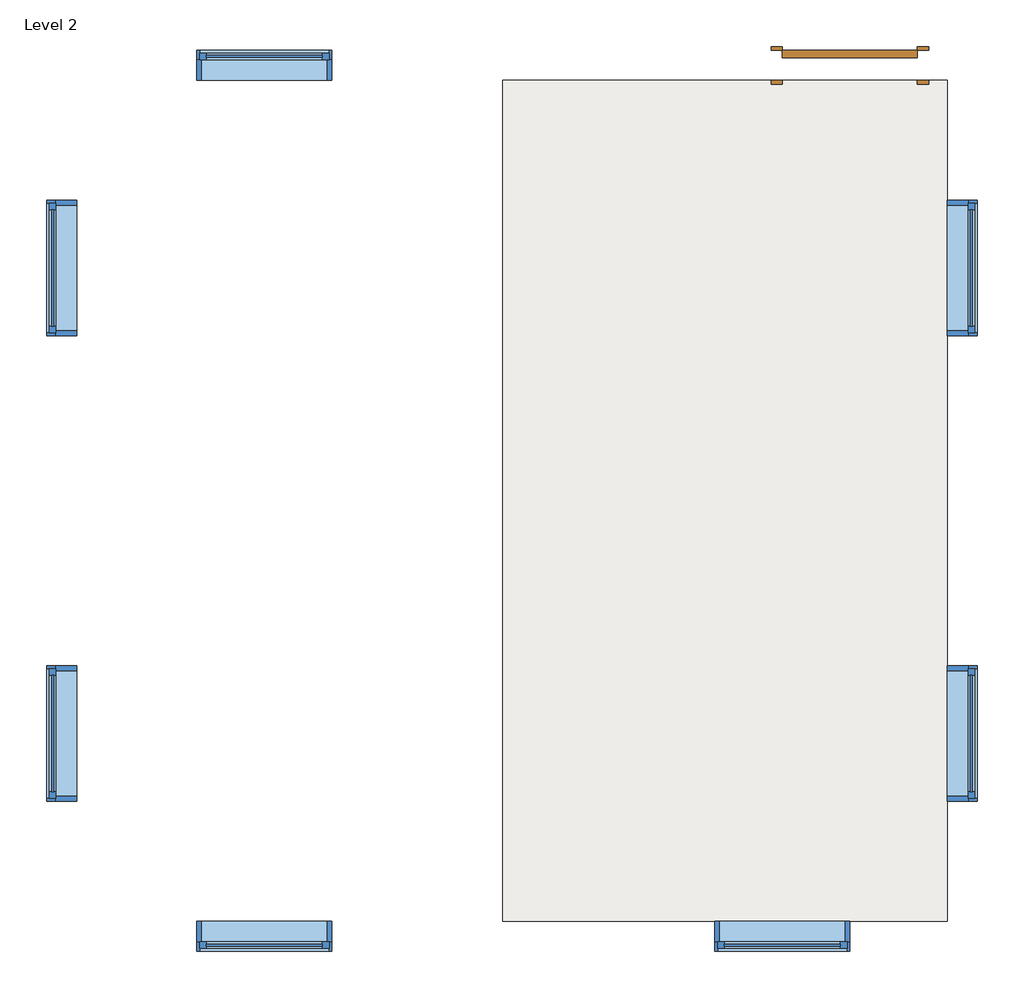
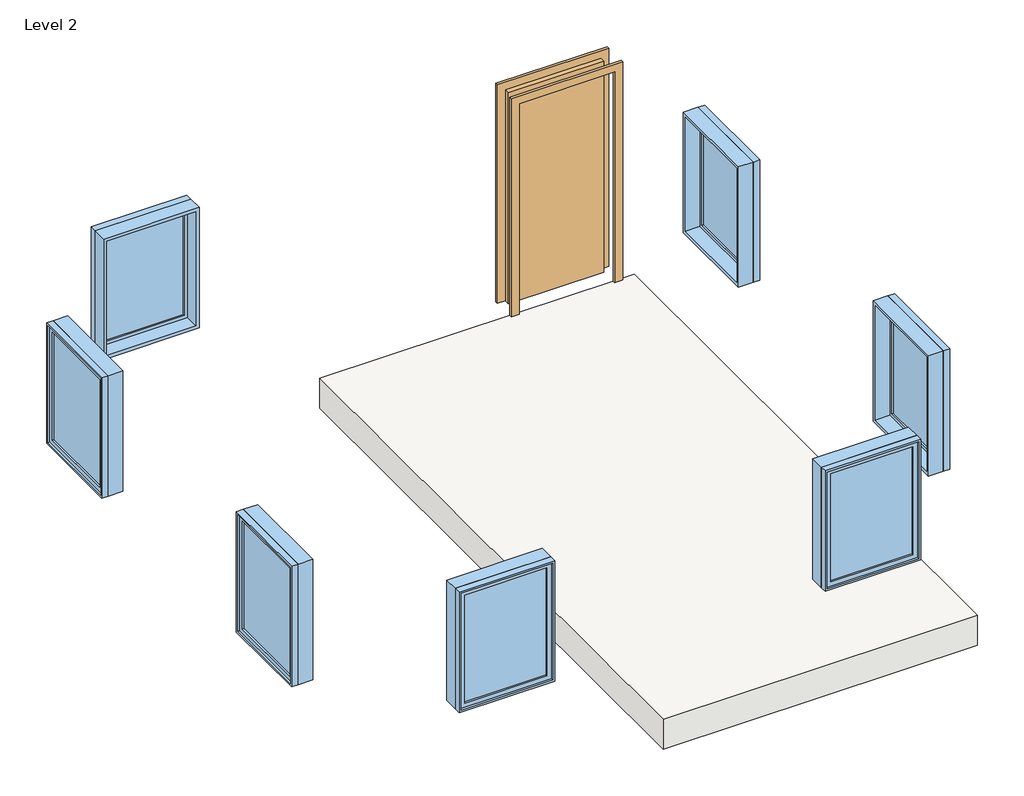
# One storey: 7 windows, 1 door, 1 slab.
"""IFC4 building model written with IfcOpenShell, lengths in millimetres."""

import ifcopenshell
import ifcopenshell.guid

model = None  # the IFC model being written
_history = None  # IfcOwnerHistory: only IFC2X3 demands one
_inside = {}  # id of a spatial element -> (the spatial element, [elements in it])
_under = {}  # id of a project, library or spatial element -> (it, [spatial elements below it])
_declared = {}  # id of a project -> (the project, [libraries it declares])
_typed = {}  # id of a type object -> (the type object, [elements of that type])
_made_of = {}  # id of a material, layer set ... -> (it, [elements and type objects made of it])


def new_model(schema):
    """Start an empty IFC model of exactly this schema.

    Asked for "IFC4X3", IfcOpenShell would pick the latest addendum, in which some entities
    have other attributes; the version numbers below select the first issue.
    IFC2X3 requires an IfcOwnerHistory on every rooted entity: one is made here for all.
    """
    global model, _history
    if schema == "IFC4X3":
        model = ifcopenshell.file(schema_version=(4, 3, 0, 0))
    else:
        model = ifcopenshell.file(schema=schema)
    _inside.clear()
    _under.clear()
    _declared.clear()
    _typed.clear()
    _made_of.clear()
    _history = None
    if model.schema == "IFC2X3":
        org = make("IfcOrganization", Name="unknown")
        user = make(
            "IfcPersonAndOrganization",
            ThePerson=make("IfcPerson", FamilyName="unknown"),
            TheOrganization=org,
        )
        app = make(
            "IfcApplication",
            ApplicationDeveloper=org,
            Version="unknown",
            ApplicationFullName="unknown",
            ApplicationIdentifier="unknown",
        )
        _history = make(
            "IfcOwnerHistory",
            OwningUser=user,
            OwningApplication=app,
            ChangeAction="ADDED",
            CreationDate=0,
        )
    return model


def make(cls, **values):
    """One entity of the class cls with the attributes given. An attribute that is None is left unset."""
    return model.create_entity(
        cls, **{name: value for name, value in values.items() if value is not None}
    )


def rooted(cls, **values):
    """An entity with a GlobalId (a new one), such as an element, a storey or a relation."""
    return make(cls, GlobalId=ifcopenshell.guid.new(), OwnerHistory=_history, **values)


def si_unit(unit_type, name, prefix=None):
    """IfcSIUnit, for example si_unit("LENGTHUNIT", "METRE", prefix="MILLI")."""
    return make("IfcSIUnit", UnitType=unit_type, Prefix=prefix, Name=name)


def assignment(units):
    """IfcUnitAssignment: the units of a project."""
    return None if units is None else make("IfcUnitAssignment", Units=units)


def point(xyz):
    """IfcCartesianPoint."""
    return None if xyz is None else make("IfcCartesianPoint", Coordinates=xyz)


def direction(xyz):
    """IfcDirection."""
    return None if xyz is None else make("IfcDirection", DirectionRatios=xyz)


def frame(location, z_axis=None, x_axis=None):
    """IfcAxis2Placement3D, a coordinate frame: its origin and axes. An axis left out is left unset."""
    return make(
        "IfcAxis2Placement3D",
        Location=point(location),
        Axis=direction(z_axis),
        RefDirection=direction(x_axis),
    )


def origin():
    """The frame at (0, 0, 0) with its axes left unset."""
    return frame((0.0, 0.0, 0.0))


def origin_with_axes():
    """The frame at (0, 0, 0) with the z axis (0, 0, 1) and the x axis (1, 0, 0) written out."""
    return frame((0.0, 0.0, 0.0), z_axis=(0.0, 0.0, 1.0), x_axis=(1.0, 0.0, 0.0))


def place(relative_to, where):
    """IfcLocalPlacement: puts the frame where relative to a parent placement (None: the world)."""
    return make(
        "IfcLocalPlacement", PlacementRelTo=relative_to, RelativePlacement=where
    )


def context(
    kind, dimensions, precision=None, world=None, true_north=None, identifier=None
):
    """IfcGeometricRepresentationContext, for example the 3D "Model" context."""
    return make(
        "IfcGeometricRepresentationContext",
        ContextIdentifier=identifier,
        ContextType=kind,
        CoordinateSpaceDimension=dimensions,
        Precision=precision,
        WorldCoordinateSystem=world,
        TrueNorth=true_north,
    )


def project(units=None, contexts=None):
    """IfcProject with its units and contexts."""
    return rooted(
        "IfcProject",
        Name="project",
        RepresentationContexts=contexts,
        UnitsInContext=assignment(units),
    )


def spatial(cls, under=None, at=None, **own):
    """A site, building, storey or space (cls), placed at a placement, below another one or the project."""
    s = rooted(cls, ObjectPlacement=at, **own)
    if under is not None:
        _under.setdefault(under.id(), (under, []))[1].append(s)
    return s


def polyline(points):
    """IfcPolyline through the points."""
    return make("IfcPolyline", Points=[point(p) for p in points])


def outline(outer, holes=None, kind="AREA"):
    """IfcArbitraryClosedProfileDef: a profile drawn as a closed curve; with holes, ...WithVoids."""
    if holes is None:
        return make("IfcArbitraryClosedProfileDef", ProfileType=kind, OuterCurve=outer)
    return make(
        "IfcArbitraryProfileDefWithVoids",
        ProfileType=kind,
        OuterCurve=outer,
        InnerCurves=holes,
    )


def extrude(swept, where, along, depth):
    """IfcExtrudedAreaSolid: the profile swept, set in the frame where, extruded along a direction by depth."""
    return make(
        "IfcExtrudedAreaSolid",
        SweptArea=swept,
        Position=where,
        ExtrudedDirection=direction(along),
        Depth=depth,
    )


def faces_of(points, faces, orient=None, outer=None):
    """IfcFace entities. A face is a list of loops; a loop is a list of indices into points, from 0.

    orient and outer hold one flag for each loop. By default every Orientation is true, the
    first loop of a face is its IfcFaceOuterBound and the others are IfcFaceBound.
    """
    made = []
    for i, loops in enumerate(faces):
        bounds = []
        for j, loop in enumerate(loops):
            is_outer = j == 0 if outer is None else outer[i][j]
            bounds.append(
                make(
                    "IfcFaceOuterBound" if is_outer else "IfcFaceBound",
                    Bound=make("IfcPolyLoop", Polygon=[points[k] for k in loop]),
                    Orientation=True if orient is None else orient[i][j],
                )
            )
        made.append(make("IfcFace", Bounds=bounds))
    return made


def faceted_brep(points, faces, orient=None, outer=None, voids=None):
    """IfcFacetedBrep: a solid bounded by flat faces; with voids (closed shells), ...WithVoids."""
    shared = [point(p) for p in points]
    hull = make("IfcClosedShell", CfsFaces=faces_of(shared, faces, orient, outer))
    if voids is None:
        return make("IfcFacetedBrep", Outer=hull)
    return make(
        "IfcFacetedBrepWithVoids",
        Outer=hull,
        Voids=[
            make(cls, CfsFaces=faces_of(shared, fs, o, b)) for cls, fs, o, b in voids
        ],
    )


def shape(context_of_items, identifier, shape_type, items):
    """IfcShapeRepresentation: the items that make up one representation, for example the "Body"."""
    return make(
        "IfcShapeRepresentation",
        ContextOfItems=context_of_items,
        RepresentationIdentifier=identifier,
        RepresentationType=shape_type,
        Items=items,
    )


def source(mapping_origin, context_of_items, identifier, shape_type, items):
    """IfcRepresentationMap: a shape defined once, which mapped items show again and again."""
    return make(
        "IfcRepresentationMap",
        MappingOrigin=mapping_origin,
        MappedRepresentation=shape(context_of_items, identifier, shape_type, items),
    )


def transform(
    local_origin,
    x_axis=None,
    y_axis=None,
    z_axis=None,
    scale=None,
    scale2=None,
    scale3=None,
    uniform=True,
):
    """IfcCartesianTransformationOperator3D, or its non-uniform kind. x_axis, y_axis, z_axis: its Axis1, 2, 3."""
    if uniform:
        return make(
            "IfcCartesianTransformationOperator3D",
            Axis1=direction(x_axis),
            Axis2=direction(y_axis),
            LocalOrigin=point(local_origin),
            Scale=scale,
            Axis3=direction(z_axis),
        )
    return make(
        "IfcCartesianTransformationOperator3DnonUniform",
        Axis1=direction(x_axis),
        Axis2=direction(y_axis),
        LocalOrigin=point(local_origin),
        Scale=scale,
        Axis3=direction(z_axis),
        Scale2=scale2,
        Scale3=scale3,
    )


def mapped(mapping_source, mapping_target):
    """IfcMappedItem: shows the shape of a source again, moved by a transform."""
    return make(
        "IfcMappedItem", MappingSource=mapping_source, MappingTarget=mapping_target
    )


def made_of(thing, what):
    """Note that an element or type object is made of a material, layer set ...; save() writes the relation."""
    if what is not None:
        _made_of.setdefault(what.id(), (what, []))[1].append(thing)
    return thing


def element(
    cls,
    number,
    at=None,
    inside=None,
    cuts=None,
    type_object=None,
    material=None,
    context=None,
    identifier="Body",
    shape_type=None,
    held_by="IfcProductDefinitionShape",
    body=None,
    shapes=None,
    **own,
):
    """One element of the class cls, such as IfcWall. Its Tag is "e" and its number.

    at: its placement. inside: the storey or other place that contains it. cuts: it is an
    opening in that element (IfcRelVoidsElement). A single representation is given by context,
    identifier, shape_type and body (its items); several are given by shapes. held_by: the class
    of the entity that holds the representations. save() writes the other relations.
    """
    e = rooted(cls, Tag="e%d" % number, ObjectPlacement=at, **own)
    if body is not None:
        shapes = [shape(context, identifier, shape_type, body)]
    if shapes is not None:
        e.Representation = make(held_by, Representations=shapes)
    if inside is not None:
        _inside.setdefault(inside.id(), (inside, []))[1].append(e)
    if cuts is not None:
        rooted(
            "IfcRelVoidsElement", RelatingBuildingElement=cuts, RelatedOpeningElement=e
        )
    if type_object is not None:
        _typed.setdefault(type_object.id(), (type_object, []))[1].append(e)
    return made_of(e, material)


def aggregate(whole, parts):
    """IfcRelAggregates: a whole, such as a stair, and the parts it consists of."""
    return rooted("IfcRelAggregates", RelatingObject=whole, RelatedObjects=parts)


def save(model, path):
    """Write the relations noted so far, then the file.

    IfcRelAggregates (storeys below a building ...), IfcRelContainedInSpatialStructure (elements
    in a storey), IfcRelDefinesByType, IfcRelAssociatesMaterial and IfcRelDeclares: one each for
    every whole, place, type object, material and project.
    """
    for whole, parts in _under.values():
        aggregate(whole, parts)
    for where, things in _inside.values():
        rooted(
            "IfcRelContainedInSpatialStructure",
            RelatedElements=things,
            RelatingStructure=where,
        )
    for kind, things in _typed.values():
        rooted("IfcRelDefinesByType", RelatedObjects=things, RelatingType=kind)
    for what, things in _made_of.values():
        rooted("IfcRelAssociatesMaterial", RelatedObjects=things, RelatingMaterial=what)
    for by, libraries in _declared.values():
        rooted("IfcRelDeclares", RelatingContext=by, RelatedDefinitions=libraries)
    model.write(path)


def door_54dd4da4(model_context):
    return source(origin(), model_context, "Body", "SweptSolid", [
        extrude(outline(polyline([(2209.8, -533.4), (0.0, -533.4), (0.0, -457.2), (2133.6, -457.2), (2133.6, 457.2), (0.0, 457.2), (0.0, 533.4), (2209.8, 533.4), (2209.8, -533.4)])), frame((0.0, 101.6, 0.0), z_axis=(0.0, 1.0, 0.0), x_axis=(0.0, 0.0, 1.0)), (0.0, 0.0, 1.0), 25.4),
        extrude(outline(polyline([(2209.8, 533.4), (2209.8, -533.4), (0.0, -533.4), (0.0, -457.2), (2133.6, -457.2), (2133.6, 457.2), (0.0, 457.2), (0.0, 533.4), (2209.8, 533.4)])), frame((0.0, -127.0, 0.0), z_axis=(0.0, 1.0, 0.0), x_axis=(0.0, 0.0, 1.0)), (0.0, 0.0, 1.0), 25.4),
        extrude(outline(polyline([(457.2, 50.8), (-457.2, 50.8), (-457.2, 101.6), (457.2, 101.6), (457.2, 50.8)])), origin_with_axes(), (0.0, 0.0, 1.0), 2133.6),
    ])


def window_e2841890(model_context):
    return source(origin(), model_context, "Body", "SweptSolid", [
        extrude(outline(polyline([(355.6, 53.975), (-431.8, 53.975), (-431.8, 66.675), (355.6, 66.675), (355.6, 53.975)])), frame((0.0, 0.0, 977.9), z_axis=(0.0, 0.0, 1.0), x_axis=(1.0, 0.0, 0.0)), (0.0, 0.0, 1.0), 1092.2),
        extrude(outline(polyline([(2114.55, -476.25), (933.45, -476.25), (933.45, 400.05), (2114.55, 400.05), (2114.55, -476.25)]), holes=[polyline([(2070.1, -431.8), (2070.1, 355.6), (977.9, 355.6), (977.9, -431.8), (2070.1, -431.8)])]), frame((0.0, 38.1, 0.0), z_axis=(0.0, 1.0, 0.0), x_axis=(0.0, 0.0, 1.0)), (0.0, 0.0, 1.0), 44.45),
        extrude(outline(polyline([(2133.6, -495.3), (914.4, -495.3), (914.4, 419.1), (2133.6, 419.1), (2133.6, -495.3)]), holes=[polyline([(2101.85, -463.55), (2101.85, 387.35), (946.15, 387.35), (946.15, -463.55), (2101.85, -463.55)])]), frame((0.0, -101.6, 0.0), z_axis=(0.0, 1.0, 0.0), x_axis=(0.0, 0.0, 1.0)), (0.0, 0.0, 1.0), 139.7),
        extrude(outline(polyline([(2133.6, 419.1), (2133.6, -495.3), (914.4, -495.3), (914.4, 419.1), (2133.6, 419.1)]), holes=[polyline([(2114.55, 400.05), (933.45, 400.05), (933.45, -476.25), (2114.55, -476.25), (2114.55, 400.05)])]), frame((0.0, 38.1, 0.0), z_axis=(0.0, 1.0, 0.0), x_axis=(0.0, 0.0, 1.0)), (0.0, 0.0, 1.0), 63.5),
    ])


model = new_model("IFC4")

# Units and contexts
model_context = context("Model", 3, world=origin())
ifc_project = project(units=[si_unit("LENGTHUNIT", "METRE", prefix="MILLI")], contexts=[model_context])

# Site, building, storey
site = spatial("IfcSite", under=ifc_project)
building = spatial("IfcBuilding", under=site)
storey = spatial("IfcBuildingStorey", under=building, Name="Level 2", Elevation=3048.0)

# Door
placement = place(None, origin())
door_shape = door_54dd4da4(model_context)
element("IfcDoor", 1, ObjectType="Single-Flush : 36\" x 84\"", at=placement, inside=storey, context=model_context, shape_type="MappedRepresentation", body=[
    mapped(door_shape, transform((16538.7123343, 13565.2483822, 3048.0), x_axis=(1.0, 0.0, 0.0), y_axis=(0.0, 1.0, 0.0), z_axis=(0.0, 0.0, 1.0))),
])

# Slab
element("IfcSlab", 2, ObjectType="Generic - 12\"", at=placement, inside=storey, context=model_context, shape_type="Brep", body=[
    faceted_brep([(17199.1123343, 13463.6483822, 2743.2), (17199.1123343, 7774.0483822, 2743.2), (14189.2123343, 7774.0483822, 2743.2), (14189.2123343, 13463.6483822, 2743.2), (17199.1123343, 13463.6483822, 3048.0), (16995.9123343, 13463.6483822, 3048.0), (16081.5123343, 13463.6483822, 3048.0), (14189.2123343, 13463.6483822, 3048.0), (14189.2123343, 7774.0483822, 3048.0), (17199.1123343, 7774.0483822, 3048.0)], [[[0, 1, 2, 3]], [[4, 5, 6, 7, 8, 9]], [[1, 0, 4, 9]], [[2, 1, 9, 8]], [[3, 2, 8, 7]], [[0, 3, 7, 6, 5, 4]]]),
])

# Windows
window_shape = window_e2841890(model_context)
element("IfcWindow", 3, ObjectType="Fixed : 36\" x 48\"", at=placement, inside=storey, context=model_context, shape_type="MappedRepresentation", body=[
    mapped(window_shape, transform((12614.4123343, 13565.2483822, 3048.0), x_axis=(1.0, 0.0, 0.0), y_axis=(0.0, 1.0, 0.0), z_axis=(0.0, 0.0, 1.0))),
])
element("IfcWindow", 4, ObjectType="Fixed : 36\" x 48\"", at=placement, inside=storey, context=model_context, shape_type="MappedRepresentation", body=[
    mapped(window_shape, transform((12538.2123343, 7672.4483822, 3048.0), x_axis=(-1.0, 0.0, 0.0), y_axis=(0.0, -1.0, 0.0), z_axis=(0.0, 0.0, 1.0))),
])
element("IfcWindow", 5, ObjectType="Fixed : 36\" x 48\"", at=placement, inside=storey, context=model_context, shape_type="MappedRepresentation", body=[
    mapped(window_shape, transform((16043.4123343, 7672.4483822, 3048.0), x_axis=(-1.0, 0.0, 0.0), y_axis=(0.0, -1.0, 0.0), z_axis=(0.0, 0.0, 1.0))),
])
element("IfcWindow", 6, ObjectType="Fixed : 36\" x 48\"", at=placement, inside=storey, context=model_context, shape_type="MappedRepresentation", body=[
    mapped(window_shape, transform((11204.7123343, 9082.1483822, 3048.0), x_axis=(0.0, 1.0, 0.0), y_axis=(-1.0, 0.0, 0.0), z_axis=(0.0, 0.0, 1.0))),
])
element("IfcWindow", 7, ObjectType="Fixed : 36\" x 48\"", at=placement, inside=storey, context=model_context, shape_type="MappedRepresentation", body=[
    mapped(window_shape, transform((11204.7123343, 12231.7483822, 3048.0), x_axis=(0.0, 1.0, 0.0), y_axis=(-1.0, 0.0, 0.0), z_axis=(0.0, 0.0, 1.0))),
])
element("IfcWindow", 8, ObjectType="Fixed : 36\" x 48\"", at=placement, inside=storey, context=model_context, shape_type="MappedRepresentation", body=[
    mapped(window_shape, transform((17300.7123343, 12155.5483822, 3048.0), x_axis=(0.0, -1.0, 0.0), y_axis=(1.0, 0.0, 0.0), z_axis=(0.0, 0.0, 1.0))),
])
element("IfcWindow", 9, ObjectType="Fixed : 36\" x 48\"", at=placement, inside=storey, context=model_context, shape_type="MappedRepresentation", body=[
    mapped(window_shape, transform((17300.7123343, 9005.9483822, 3048.0), x_axis=(0.0, -1.0, 0.0), y_axis=(1.0, 0.0, 0.0), z_axis=(0.0, 0.0, 1.0))),
])

save(model, "model.ifc")

# Revit data of these elements
# Type "Single-Flush : 36\" x 84\""
#   Type Mark = "1"
#   Construction Type Id = "MDOOR"
#   Assembly Code = "C1020"
#   Analytic Construction = "Metal"
#   Thickness = 0' - 2"
#   Heat Transfer Coefficient (U) = 0.651978 BTU/(h·ft²·°F)
#   Height = 7' - 0"
#   Trim Projection Ext = 0' - 1"
#   Trim Projection Int = 0' - 1"
#   Trim Width = 0' - 3"
#   Width = 3' - 0"
#   Define Thermal Properties by = 1
#   Door Material = Door - Panel
#   Frame Material = Door - Frame
#   Visual Light Transmittance = 0
#   Solar Heat Gain Coefficient = 0
#   Function = (empty or 0)
#   Wall Closure = (empty or 0)
# Type "Generic - 12\""
#   Assembly Code = "B1010"
#   Function = 0
#   Layers, outside or top first: 1' - 0" no material (function 1)
# Type "Fixed : 36\" x 48\""
#   Type Mark = "1"
#   Construction Type Id = "GSP4R"
#   Assembly Code = "B2020100"
#   Analytic Construction = "1/8 in Pilkington single glazing"
#   Visual Light Transmittance = 0.9
#   Solar Heat Gain Coefficient = 0.78
#   Heat Transfer Coefficient (U) = 0.6496 BTU/(h·ft²·°F)
#   Height = 4' - 0"
#   Default Sill Height = 3' - 0"
#   Width = 3' - 0"
#   Window Inset = 0' - 0 3/4"
#   Define Thermal Properties by = 1
#   Glass Pane Material = Glass
#   Sash Material = Sash
#   Wall Closure = (empty or 0)
# Element 1 (IfcDoor, "Single-Flush : 36\" x 84\"")
#   Phase Created = New Construction
#   Materials on its faces: "Door - Frame", "Door - Panel"
# Element 2 (IfcSlab, "Generic - 12\"")
#   Height Offset From Level = 0' - 0"
#   Phase Created = New Construction
#   Materials on its faces: "Default Floor"
# Element 3 (IfcWindow, "Fixed : 36\" x 48\"")
#   Mark = "4"
#   Phase Created = New Construction
#   Materials on its faces: "Sash", "Glass"
# Element 4 (IfcWindow, "Fixed : 36\" x 48\"")
#   Mark = "5"
#   Phase Created = New Construction
#   Materials on its faces: "Sash", "Glass"
# Element 5 (IfcWindow, "Fixed : 36\" x 48\"")
#   Mark = "6"
#   Phase Created = New Construction
#   Materials on its faces: "Sash", "Glass"
# Element 6 (IfcWindow, "Fixed : 36\" x 48\"")
#   Mark = "7"
#   Phase Created = New Construction
#   Materials on its faces: "Sash", "Glass"
# Element 7 (IfcWindow, "Fixed : 36\" x 48\"")
#   Mark = "8"
#   Phase Created = New Construction
#   Materials on its faces: "Sash", "Glass"
# Element 8 (IfcWindow, "Fixed : 36\" x 48\"")
#   Mark = "9"
#   Phase Created = New Construction
#   Materials on its faces: "Sash", "Glass"
# Element 9 (IfcWindow, "Fixed : 36\" x 48\"")
#   Mark = "10"
#   Phase Created = New Construction
#   Materials on its faces: "Sash", "Glass"
# Materials
#   "Door - Panel": class "Wood", colour RGB 210 159 95, transparency 0
#   "Door - Frame": class "Miscellaneous", colour RGB 118 70 51, transparency 0
#   "Glass": class "Glass", colour RGB 0 128 192, transparency 0.75, Description = "Soda Lime Glass", Cost = 0
#   "Sash": class "Wood", colour RGB 224 178 126, transparency 0
#   "Default Floor": class "Miscellaneous", colour RGB 128 128 128, transparency 0
